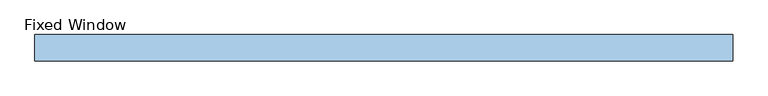
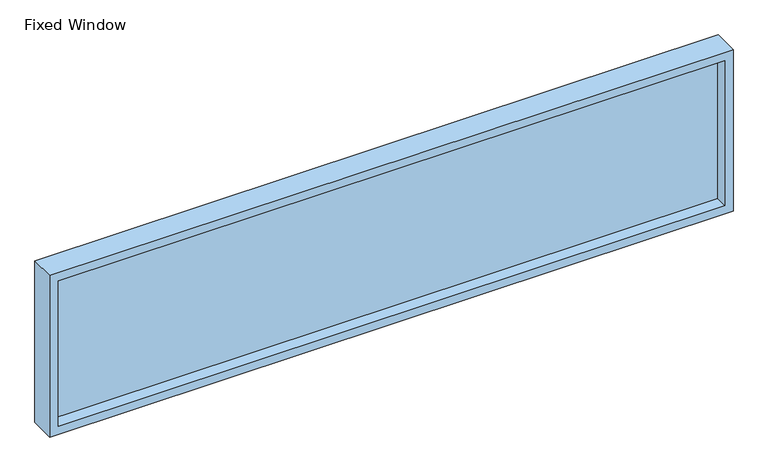
"""IFC4 building model written with IfcOpenShell, lengths in millimetres: window geometry, Fixed Window : H_WD_AMW_AL Window_DG_W4000xH1000_Fixed_1H1V."""

from ifc_helpers import new_model, si_unit, frame, origin, place, context, project, spatial, polyline, outline, extrude, source, transform, mapped, element, save


def fixed_window_3ff382ba(model_context):
    return source(origin(), model_context, "Body", "SweptSolid", [
        extrude(outline(polyline([(-1950.0, 3.0), (1950.0, 3.0), (1950.0, -3.0), (-1950.0, -3.0), (-1950.0, 3.0)])), frame((0.0, 0.0, 850.0), z_axis=(0.0, 0.0, 1.0), x_axis=(1.0, 0.0, 0.0)), (0.0, 0.0, 1.0), 900.0),
        extrude(outline(polyline([(1800.0, -2000.0), (800.0, -2000.0), (800.0, 2000.0), (1800.0, 2000.0), (1800.0, -2000.0)]), holes=[polyline([(1750.0, -1950.0), (1750.0, 1950.0), (850.0, 1950.0), (850.0, -1950.0), (1750.0, -1950.0)])]), frame((0.0, -75.0, 0.0), z_axis=(0.0, 1.0, 0.0), x_axis=(0.0, 0.0, 1.0)), (0.0, 0.0, 1.0), 150.0),
    ])


if __name__ == "__main__":
    model = new_model("IFC4")
    model_context = context("Model", 3, world=origin())
    ifc_project = project(units=[si_unit("LENGTHUNIT", "METRE", prefix="MILLI")], contexts=[model_context])
    site = spatial("IfcSite", under=ifc_project)
    building = spatial("IfcBuilding", under=site)
    placement = place(None, origin())
    fixed_window_shape = fixed_window_3ff382ba(model_context)
    element("IfcWindow", 1, ObjectType="Fixed Window : H_WD_AMW_AL Window_DG_W4000xH1000_Fixed_1H1V", at=placement, inside=building, context=model_context, shape_type="MappedRepresentation", body=[
        mapped(fixed_window_shape, transform((0.0, 0.0, 0.0), x_axis=(1.0, 0.0, 0.0), y_axis=(0.0, 1.0, 0.0), z_axis=(0.0, 0.0, 1.0))),
    ])
    save(model, "model.ifc")

# Revit data of these elements
# Type "Fixed Window : H_WD_AMW_AL Window_DG_W4000xH1000_Fixed_1H1V"
#   Type Mark = "AW"
#   H_WM Code_1 = "A04AR159-00001 | Finishing Work | Door & Window Work | Aluminum Window (UoM: EA) | Fire Protective Rating: N/A | w/ Hardware & Accessories | W x H=(  )mm x (  )mm"
#   H_Q'ty Cal Type Tag = "WD-Q1"
#   Analytic Construction = "<None>"
#   창 두께 = 0.1500 m
#   Height = 1.0000 m
#   절반 창 두께 = 0.0750 m
#   기본 씰 높이 = 0.8000 m
#   Width = 4.0000 m
#   Wall Closure = 3
#   Define Thermal Properties by = 1
#   창 패널 = AW2 창 패널
#   창 프레임 = A04AQ127-00002_Aluminum Window_None FP
#   Description = (empty or 0)
# Element 1 (IfcWindow, "Fixed Window : H_WD_AMW_AL Window_DG_W4000xH1000_Fixed_1H1V")
#   Materials on its faces: "A04AQ127-00002_Aluminum Window_None FP", "AW2 창 패널"
# Materials
#   "AW2 창 패널": class "유리", colour RGB 0 0 255, transparency 0.75
#   "A04AQ127-00002_Aluminum Window_None FP": class "금속", colour RGB 247 247 247, transparency 0, Cost = 0
